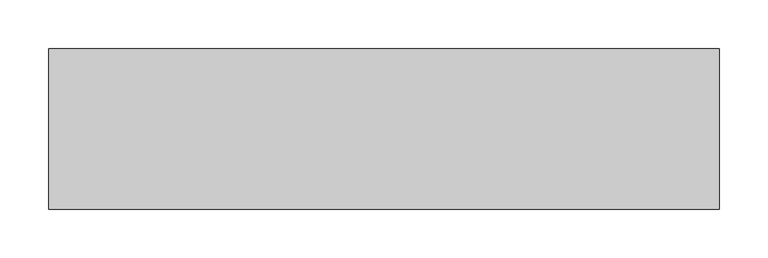
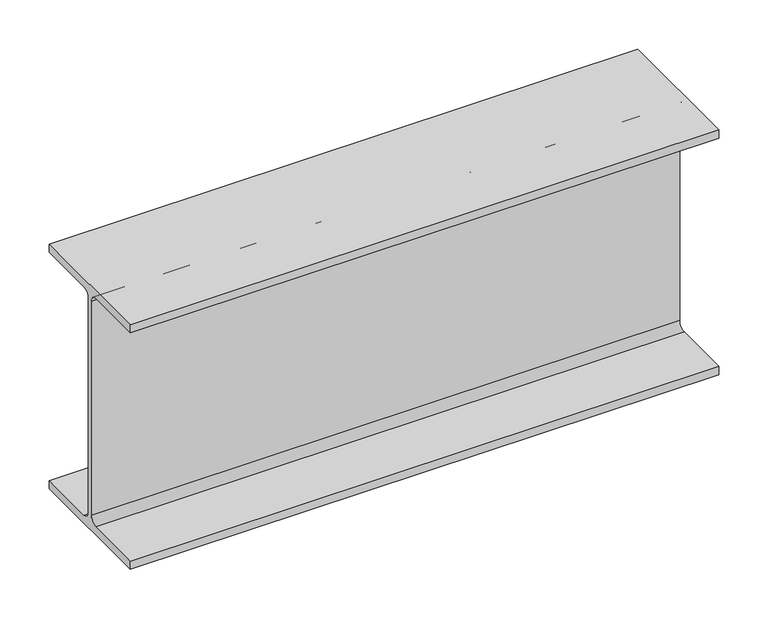
"""IFC4 building model written with IfcOpenShell, lengths in millimetres: beam geometry, Steel Beam_H-KSD3502 : H_SB_ASB_H-300x150x6.5x9."""

from ifc_helpers import new_model, si_unit, point, frame, frame_2d, origin, place, context, project, spatial, polyline, circle_curve, trimmed, segment, composite_curve, outline, extrude, source, transform, mapped, element, save


def beam_6268a929(model_context):
    return source(origin(), model_context, "Body", "SweptSolid", [
        extrude(outline(composite_curve([segment(polyline([(82.5, -141.5), (82.5, -151.7), (-82.5, -151.7), (-82.5, -141.5), (-11.9, -141.5)]), True, "CONTINUOUS"), segment(trimmed(circle_curve(frame_2d((-11.9, -132.6)), 8.9), [point((-11.9, -141.5))], [point((-3.0, -132.6))], True, "CARTESIAN"), True, "CONTINUOUS"), segment(polyline([(-3.0, -132.6), (-3.0, 132.6)]), True, "CONTINUOUS"), segment(trimmed(circle_curve(frame_2d((-11.9, 132.6)), 8.9), [point((-3.0, 132.6))], [point((-11.9, 141.5))], True, "CARTESIAN"), True, "CONTINUOUS"), segment(polyline([(-11.9, 141.5), (-82.5, 141.5), (-82.5, 151.7), (82.5, 151.7), (82.5, 141.5), (11.9, 141.5)]), True, "CONTINUOUS"), segment(trimmed(circle_curve(frame_2d((11.9, 132.6)), 8.9), [point((11.9, 141.5))], [point((3.0, 132.6))], True, "CARTESIAN"), True, "CONTINUOUS"), segment(polyline([(3.0, 132.6), (3.0, -132.6)]), True, "CONTINUOUS"), segment(trimmed(circle_curve(frame_2d((11.9, -132.6)), 8.9), [point((3.0, -132.6))], [point((11.9, -141.5))], True, "CARTESIAN"), True, "CONTINUOUS"), segment(polyline([(11.9, -141.5), (82.5, -141.5)]), True, "CONTINUOUS")], self_intersect=False)), frame((-345.0, 0.0, 0.0), z_axis=(1.0, 0.0, 0.0), x_axis=(0.0, 1.0, 0.0)), (0.0, 0.0, 1.0), 689.9999994),
    ])


if __name__ == "__main__":
    model = new_model("IFC4")
    model_context = context("Model", 3, world=origin())
    ifc_project = project(units=[si_unit("LENGTHUNIT", "METRE", prefix="MILLI")], contexts=[model_context])
    site = spatial("IfcSite", under=ifc_project)
    building = spatial("IfcBuilding", under=site)
    placement = place(None, origin())
    beam_shape = beam_6268a929(model_context)
    element("IfcBeam", 1, ObjectType="Steel Beam_H-KSD3502 : H_SB_ASB_H-300x150x6.5x9", at=placement, inside=building, context=model_context, shape_type="MappedRepresentation", body=[
        mapped(beam_shape, transform((0.0, 0.0, 0.0), x_axis=(1.0, 0.0, 0.0), y_axis=(0.0, 1.0, 0.0), z_axis=(0.0, 0.0, 1.0))),
    ])
    save(model, "model.ifc")

# Revit data of these elements
# Type "Steel Beam_H-KSD3502 : H_SB_ASB_H-300x150x6.5x9"
#   Width = 15.0 cm
#   Web Thickness = 0.65 cm
#   Web Fillet = 1.3 cm
#   Warping Constant = 107174.0 cm⁶
#   Torsional Moment of Inertia = 9.9539 cm⁴
#   Torsional Modulus = 1.0 cm³
#   Section Area = 46.78 cm²
#   Plastic Modulus weak axis = 105.0 cm³
#   Plastic Modulus strong axis = 542.0 cm³
#   Perimeter = 1.17 m²/m
#   Nominal Weight = 36.70 kgf/m
#   Moment of Inertia weak axis = 508.00 cm⁴
#   Moment of Inertia strong axis = 7210.00 cm⁴
#   Height = 30.0 cm
#   Flange Thickness = 0.9 cm
#   Elastic Modulus weak axis = 67.7 cm³
#   Elastic Modulus strong axis = 481.0 cm³
#   Centroid Vertical = 15.0 cm
#   Centroid Horizontal = 7.5 cm
#   Length [instance default] = 1.5240 m
#   Structural Material [instance default] = Steel, 45-345
#   Assembly Code = ""
# Element 1 (IfcBeam, "Steel Beam_H-KSD3502 : H_SB_ASB_H-300x150x6.5x9")
#   Structural Material = none
# Materials
#   "Steel, 45-345": class "Metal", colour RGB 189 187 185, transparency 0, Description = "Steel 345 MPa", Cost = 0
